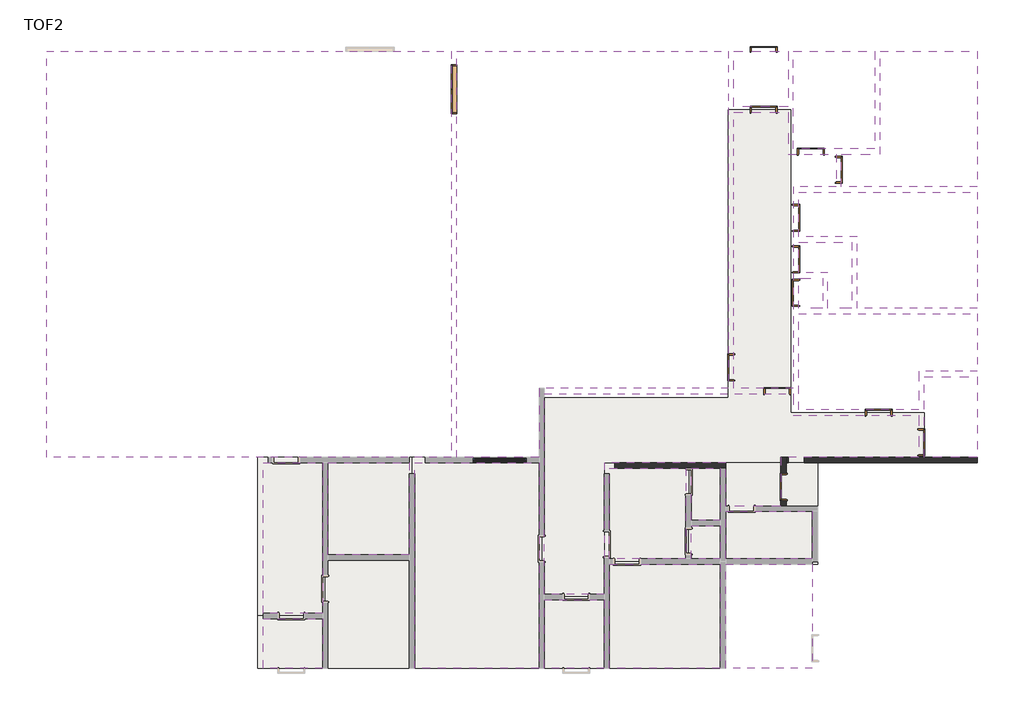
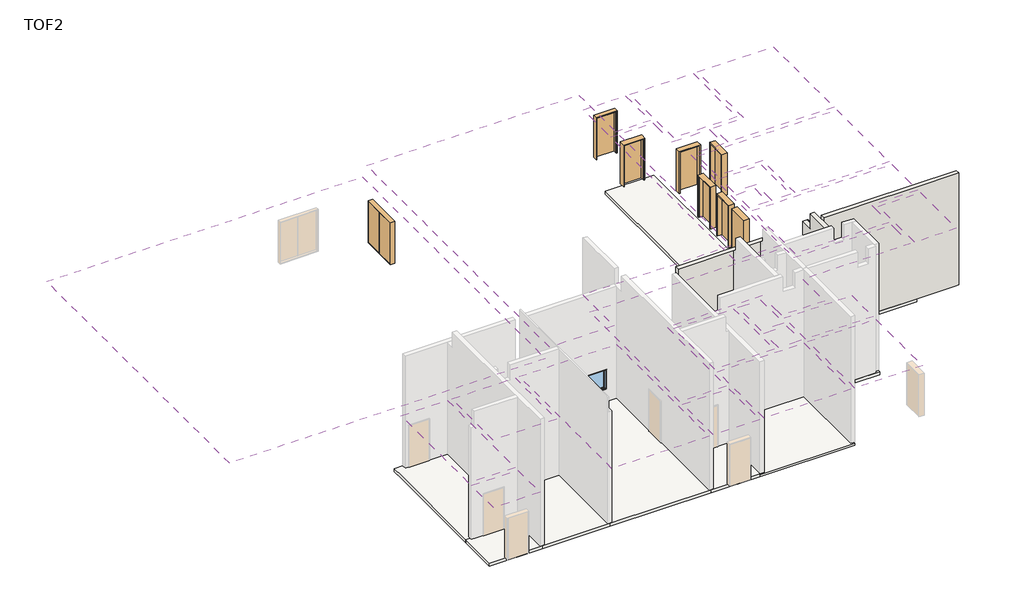
# One storey, part 2 of 2: 23 coverings, 13 doors, 12 slabs, 3 walls, 1 window.
"""IFC4 building model written with IfcOpenShell, lengths in millimetres."""

import ifcopenshell
import ifcopenshell.guid

model = None  # the IFC model being written
_history = None  # IfcOwnerHistory: only IFC2X3 demands one
_inside = {}  # id of a spatial element -> (the spatial element, [elements in it])
_under = {}  # id of a project, library or spatial element -> (it, [spatial elements below it])
_declared = {}  # id of a project -> (the project, [libraries it declares])
_typed = {}  # id of a type object -> (the type object, [elements of that type])
_made_of = {}  # id of a material, layer set ... -> (it, [elements and type objects made of it])


def new_model(schema):
    """Start an empty IFC model of exactly this schema.

    Asked for "IFC4X3", IfcOpenShell would pick the latest addendum, in which some entities
    have other attributes; the version numbers below select the first issue.
    IFC2X3 requires an IfcOwnerHistory on every rooted entity: one is made here for all.
    """
    global model, _history
    if schema == "IFC4X3":
        model = ifcopenshell.file(schema_version=(4, 3, 0, 0))
    else:
        model = ifcopenshell.file(schema=schema)
    _inside.clear()
    _under.clear()
    _declared.clear()
    _typed.clear()
    _made_of.clear()
    _history = None
    if model.schema == "IFC2X3":
        org = make("IfcOrganization", Name="unknown")
        user = make(
            "IfcPersonAndOrganization",
            ThePerson=make("IfcPerson", FamilyName="unknown"),
            TheOrganization=org,
        )
        app = make(
            "IfcApplication",
            ApplicationDeveloper=org,
            Version="unknown",
            ApplicationFullName="unknown",
            ApplicationIdentifier="unknown",
        )
        _history = make(
            "IfcOwnerHistory",
            OwningUser=user,
            OwningApplication=app,
            ChangeAction="ADDED",
            CreationDate=0,
        )
    return model


def make(cls, **values):
    """One entity of the class cls with the attributes given. An attribute that is None is left unset."""
    return model.create_entity(
        cls, **{name: value for name, value in values.items() if value is not None}
    )


def rooted(cls, **values):
    """An entity with a GlobalId (a new one), such as an element, a storey or a relation."""
    return make(cls, GlobalId=ifcopenshell.guid.new(), OwnerHistory=_history, **values)


def si_unit(unit_type, name, prefix=None):
    """IfcSIUnit, for example si_unit("LENGTHUNIT", "METRE", prefix="MILLI")."""
    return make("IfcSIUnit", UnitType=unit_type, Prefix=prefix, Name=name)


def assignment(units):
    """IfcUnitAssignment: the units of a project."""
    return None if units is None else make("IfcUnitAssignment", Units=units)


def point(xyz):
    """IfcCartesianPoint."""
    return None if xyz is None else make("IfcCartesianPoint", Coordinates=xyz)


def direction(xyz):
    """IfcDirection."""
    return None if xyz is None else make("IfcDirection", DirectionRatios=xyz)


def frame(location, z_axis=None, x_axis=None):
    """IfcAxis2Placement3D, a coordinate frame: its origin and axes. An axis left out is left unset."""
    return make(
        "IfcAxis2Placement3D",
        Location=point(location),
        Axis=direction(z_axis),
        RefDirection=direction(x_axis),
    )


def origin():
    """The frame at (0, 0, 0) with its axes left unset."""
    return frame((0.0, 0.0, 0.0))


def origin_with_axes():
    """The frame at (0, 0, 0) with the z axis (0, 0, 1) and the x axis (1, 0, 0) written out."""
    return frame((0.0, 0.0, 0.0), z_axis=(0.0, 0.0, 1.0), x_axis=(1.0, 0.0, 0.0))


def place(relative_to, where):
    """IfcLocalPlacement: puts the frame where relative to a parent placement (None: the world)."""
    return make(
        "IfcLocalPlacement", PlacementRelTo=relative_to, RelativePlacement=where
    )


def context(
    kind, dimensions, precision=None, world=None, true_north=None, identifier=None
):
    """IfcGeometricRepresentationContext, for example the 3D "Model" context."""
    return make(
        "IfcGeometricRepresentationContext",
        ContextIdentifier=identifier,
        ContextType=kind,
        CoordinateSpaceDimension=dimensions,
        Precision=precision,
        WorldCoordinateSystem=world,
        TrueNorth=true_north,
    )


def project(units=None, contexts=None):
    """IfcProject with its units and contexts."""
    return rooted(
        "IfcProject",
        Name="project",
        RepresentationContexts=contexts,
        UnitsInContext=assignment(units),
    )


def spatial(cls, under=None, at=None, **own):
    """A site, building, storey or space (cls), placed at a placement, below another one or the project."""
    s = rooted(cls, ObjectPlacement=at, **own)
    if under is not None:
        _under.setdefault(under.id(), (under, []))[1].append(s)
    return s


def polyline(points):
    """IfcPolyline through the points."""
    return make("IfcPolyline", Points=[point(p) for p in points])


def outline(outer, holes=None, kind="AREA"):
    """IfcArbitraryClosedProfileDef: a profile drawn as a closed curve; with holes, ...WithVoids."""
    if holes is None:
        return make("IfcArbitraryClosedProfileDef", ProfileType=kind, OuterCurve=outer)
    return make(
        "IfcArbitraryProfileDefWithVoids",
        ProfileType=kind,
        OuterCurve=outer,
        InnerCurves=holes,
    )


def extrude(swept, where, along, depth):
    """IfcExtrudedAreaSolid: the profile swept, set in the frame where, extruded along a direction by depth."""
    return make(
        "IfcExtrudedAreaSolid",
        SweptArea=swept,
        Position=where,
        ExtrudedDirection=direction(along),
        Depth=depth,
    )


def faces_of(points, faces, orient=None, outer=None):
    """IfcFace entities. A face is a list of loops; a loop is a list of indices into points, from 0.

    orient and outer hold one flag for each loop. By default every Orientation is true, the
    first loop of a face is its IfcFaceOuterBound and the others are IfcFaceBound.
    """
    made = []
    for i, loops in enumerate(faces):
        bounds = []
        for j, loop in enumerate(loops):
            is_outer = j == 0 if outer is None else outer[i][j]
            bounds.append(
                make(
                    "IfcFaceOuterBound" if is_outer else "IfcFaceBound",
                    Bound=make("IfcPolyLoop", Polygon=[points[k] for k in loop]),
                    Orientation=True if orient is None else orient[i][j],
                )
            )
        made.append(make("IfcFace", Bounds=bounds))
    return made


def faceted_brep(points, faces, orient=None, outer=None, voids=None):
    """IfcFacetedBrep: a solid bounded by flat faces; with voids (closed shells), ...WithVoids."""
    shared = [point(p) for p in points]
    hull = make("IfcClosedShell", CfsFaces=faces_of(shared, faces, orient, outer))
    if voids is None:
        return make("IfcFacetedBrep", Outer=hull)
    return make(
        "IfcFacetedBrepWithVoids",
        Outer=hull,
        Voids=[
            make(cls, CfsFaces=faces_of(shared, fs, o, b)) for cls, fs, o, b in voids
        ],
    )


def shape(context_of_items, identifier, shape_type, items):
    """IfcShapeRepresentation: the items that make up one representation, for example the "Body"."""
    return make(
        "IfcShapeRepresentation",
        ContextOfItems=context_of_items,
        RepresentationIdentifier=identifier,
        RepresentationType=shape_type,
        Items=items,
    )


def source(mapping_origin, context_of_items, identifier, shape_type, items):
    """IfcRepresentationMap: a shape defined once, which mapped items show again and again."""
    return make(
        "IfcRepresentationMap",
        MappingOrigin=mapping_origin,
        MappedRepresentation=shape(context_of_items, identifier, shape_type, items),
    )


def transform(
    local_origin,
    x_axis=None,
    y_axis=None,
    z_axis=None,
    scale=None,
    scale2=None,
    scale3=None,
    uniform=True,
):
    """IfcCartesianTransformationOperator3D, or its non-uniform kind. x_axis, y_axis, z_axis: its Axis1, 2, 3."""
    if uniform:
        return make(
            "IfcCartesianTransformationOperator3D",
            Axis1=direction(x_axis),
            Axis2=direction(y_axis),
            LocalOrigin=point(local_origin),
            Scale=scale,
            Axis3=direction(z_axis),
        )
    return make(
        "IfcCartesianTransformationOperator3DnonUniform",
        Axis1=direction(x_axis),
        Axis2=direction(y_axis),
        LocalOrigin=point(local_origin),
        Scale=scale,
        Axis3=direction(z_axis),
        Scale2=scale2,
        Scale3=scale3,
    )


def mapped(mapping_source, mapping_target):
    """IfcMappedItem: shows the shape of a source again, moved by a transform."""
    return make(
        "IfcMappedItem", MappingSource=mapping_source, MappingTarget=mapping_target
    )


def made_of(thing, what):
    """Note that an element or type object is made of a material, layer set ...; save() writes the relation."""
    if what is not None:
        _made_of.setdefault(what.id(), (what, []))[1].append(thing)
    return thing


def element(
    cls,
    number,
    at=None,
    inside=None,
    cuts=None,
    type_object=None,
    material=None,
    context=None,
    identifier="Body",
    shape_type=None,
    held_by="IfcProductDefinitionShape",
    body=None,
    shapes=None,
    **own,
):
    """One element of the class cls, such as IfcWall. Its Tag is "e" and its number.

    at: its placement. inside: the storey or other place that contains it. cuts: it is an
    opening in that element (IfcRelVoidsElement). A single representation is given by context,
    identifier, shape_type and body (its items); several are given by shapes. held_by: the class
    of the entity that holds the representations. save() writes the other relations.
    """
    e = rooted(cls, Tag="e%d" % number, ObjectPlacement=at, **own)
    if body is not None:
        shapes = [shape(context, identifier, shape_type, body)]
    if shapes is not None:
        e.Representation = make(held_by, Representations=shapes)
    if inside is not None:
        _inside.setdefault(inside.id(), (inside, []))[1].append(e)
    if cuts is not None:
        rooted(
            "IfcRelVoidsElement", RelatingBuildingElement=cuts, RelatedOpeningElement=e
        )
    if type_object is not None:
        _typed.setdefault(type_object.id(), (type_object, []))[1].append(e)
    return made_of(e, material)


def aggregate(whole, parts):
    """IfcRelAggregates: a whole, such as a stair, and the parts it consists of."""
    return rooted("IfcRelAggregates", RelatingObject=whole, RelatedObjects=parts)


def save(model, path):
    """Write the relations noted so far, then the file.

    IfcRelAggregates (storeys below a building ...), IfcRelContainedInSpatialStructure (elements
    in a storey), IfcRelDefinesByType, IfcRelAssociatesMaterial and IfcRelDeclares: one each for
    every whole, place, type object, material and project.
    """
    for whole, parts in _under.values():
        aggregate(whole, parts)
    for where, things in _inside.values():
        rooted(
            "IfcRelContainedInSpatialStructure",
            RelatedElements=things,
            RelatingStructure=where,
        )
    for kind, things in _typed.values():
        rooted("IfcRelDefinesByType", RelatedObjects=things, RelatingType=kind)
    for what, things in _made_of.values():
        rooted("IfcRelAssociatesMaterial", RelatedObjects=things, RelatingMaterial=what)
    for by, libraries in _declared.values():
        rooted("IfcRelDeclares", RelatingContext=by, RelatedDefinitions=libraries)
    model.write(path)


def double_door_steel_22a565f0(model_context):
    return source(origin(), model_context, "Body", "SolidModel", [
        extrude(outline(polyline([(880.0, 60.0), (0.0, 60.0), (0.0, 100.0), (880.0, 100.0), (880.0, 60.0)])), frame((0.0, 0.0, 20.0), z_axis=(0.0, 0.0, 1.0), x_axis=(1.0, 0.0, 0.0)), (0.0, 0.0, 1.0), 2060.0),
        extrude(outline(polyline([(0.0, 60.0), (-880.0, 60.0), (-880.0, 100.0), (0.0, 100.0), (0.0, 60.0)])), frame((0.0, 0.0, 20.0), z_axis=(0.0, 0.0, 1.0), x_axis=(1.0, 0.0, 0.0)), (0.0, 0.0, 1.0), 2060.0),
        faceted_brep([(900.0, -100.0, 2100.0), (900.0, 100.0, 2100.0), (-900.0, 100.0, 2100.0), (-900.0, -100.0, 2100.0), (865.0, 60.0, 2065.0), (865.0, -100.0, 2065.0), (-865.0, -100.0, 2065.0), (-865.0, 60.0, 2065.0), (880.0, 100.0, 2080.0), (880.0, 60.0, 2080.0), (-880.0, 60.0, 2080.0), (-880.0, 100.0, 2080.0), (-900.0, 100.0, 0.0), (-900.0, -100.0, 0.0), (-865.0, -100.0, 35.0), (-865.0, 60.0, 35.0), (-880.0, 60.0, 20.0), (-880.0, 100.0, 20.0), (900.0, 100.0, 0.0), (880.0, 100.0, 20.0), (900.0, -100.0, 0.0), (865.0, -100.0, 35.0), (865.0, 60.0, 35.0), (880.0, 60.0, 20.0)], [[[0, 1, 2, 3]], [[4, 5, 6, 7]], [[8, 9, 10, 11]], [[3, 2, 12, 13]], [[7, 6, 14, 15]], [[11, 10, 16, 17]], [[18, 12, 2, 1], [8, 11, 17, 19]], [[13, 12, 18, 20]], [[0, 3, 13, 20], [21, 14, 6, 5]], [[15, 14, 21, 22]], [[23, 16, 10, 9], [4, 7, 15, 22]], [[17, 16, 23, 19]], [[20, 18, 1, 0]], [[22, 21, 5, 4]], [[19, 23, 9, 8]]]),
    ])


def single_door_steel_02f153ad(model_context):
    return source(origin(), model_context, "Body", "SolidModel", [
        extrude(outline(polyline([(470.0, -130.0), (-470.0, -130.0), (-470.0, -95.0), (470.0, -95.0), (470.0, -130.0)])), origin_with_axes(), (0.0, 0.0, 1.0), 2070.0),
        faceted_brep([(470.0, -130.0, 0.0), (470.0, -95.0, 0.0), (450.0, -95.0, 0.0), (450.0, 95.0, 0.0), (470.0, 95.0, 0.0), (470.0, 130.0, 0.0), (500.0, 130.0, 0.0), (500.0, -130.0, 0.0), (500.0, -130.0, 2100.0), (-500.0, -130.0, 2100.0), (-500.0, -130.0, 0.0), (-470.0, -130.0, 0.0), (-470.0, -130.0, 2070.0), (470.0, -130.0, 2070.0), (500.0, 130.0, 2100.0), (470.0, 130.0, 2070.0), (-470.0, 130.0, 2070.0), (-470.0, 130.0, 0.0), (-500.0, 130.0, 0.0), (-500.0, 130.0, 2100.0), (470.0, 95.0, 2070.0), (450.0, 95.0, 2050.0), (-450.0, 95.0, 2050.0), (-450.0, 95.0, 0.0), (-470.0, 95.0, 0.0), (-470.0, 95.0, 2070.0), (450.0, -95.0, 2050.0), (470.0, -95.0, 2070.0), (-470.0, -95.0, 2070.0), (-470.0, -95.0, 0.0), (-450.0, -95.0, 0.0), (-450.0, -95.0, 2050.0)], [[[0, 1, 2, 3, 4, 5, 6, 7]], [[7, 8, 9, 10, 11, 12, 13, 0]], [[6, 14, 8, 7]], [[5, 15, 16, 17, 18, 19, 14, 6]], [[4, 20, 15, 5]], [[3, 21, 22, 23, 24, 25, 20, 4]], [[2, 26, 21, 3]], [[1, 27, 28, 29, 30, 31, 26, 2]], [[0, 13, 27, 1]], [[12, 11, 29, 28]], [[11, 10, 18, 17, 24, 23, 30, 29]], [[19, 18, 10, 9]], [[25, 24, 17, 16]], [[31, 30, 23, 22]], [[14, 19, 9, 8]], [[20, 25, 16, 15]], [[26, 31, 22, 21]], [[13, 12, 28, 27]]]),
    ])


def single_door_steel_4a6c7de9(model_context):
    return source(origin(), model_context, "Body", "SolidModel", [
        extrude(outline(polyline([(470.0, 130.0), (470.0, 95.0), (-470.0, 95.0), (-470.0, 130.0), (470.0, 130.0)])), origin_with_axes(), (0.0, 0.0, 1.0), 2070.0),
        faceted_brep([(470.0, 130.0, 0.0), (500.0, 130.0, 0.0), (500.0, -130.0, 0.0), (470.0, -130.0, 0.0), (470.0, -95.0, 0.0), (450.0, -95.0, 0.0), (450.0, 95.0, 0.0), (470.0, 95.0, 0.0), (470.0, 130.0, 2070.0), (-470.0, 130.0, 2070.0), (-470.0, 130.0, 0.0), (-500.0, 130.0, 0.0), (-500.0, 130.0, 2100.0), (500.0, 130.0, 2100.0), (500.0, -130.0, 2100.0), (-500.0, -130.0, 2100.0), (-500.0, -130.0, 0.0), (-470.0, -130.0, 0.0), (-470.0, -130.0, 2070.0), (470.0, -130.0, 2070.0), (470.0, -95.0, 2070.0), (-470.0, -95.0, 2070.0), (-470.0, -95.0, 0.0), (-450.0, -95.0, 0.0), (-450.0, -95.0, 2050.0), (450.0, -95.0, 2050.0), (450.0, 95.0, 2050.0), (-450.0, 95.0, 2050.0), (-450.0, 95.0, 0.0), (-470.0, 95.0, 0.0), (-470.0, 95.0, 2070.0), (470.0, 95.0, 2070.0)], [[[0, 1, 2, 3, 4, 5, 6, 7]], [[1, 0, 8, 9, 10, 11, 12, 13]], [[2, 1, 13, 14]], [[3, 2, 14, 15, 16, 17, 18, 19]], [[4, 3, 19, 20]], [[5, 4, 20, 21, 22, 23, 24, 25]], [[6, 5, 25, 26]], [[7, 6, 26, 27, 28, 29, 30, 31]], [[0, 7, 31, 8]], [[9, 30, 29, 10]], [[10, 29, 28, 23, 22, 17, 16, 11]], [[15, 12, 11, 16]], [[21, 18, 17, 22]], [[27, 24, 23, 28]], [[14, 13, 12, 15]], [[20, 19, 18, 21]], [[26, 25, 24, 27]], [[8, 31, 30, 9]]]),
    ])


def single_door_steel_8d57826b(model_context):
    return source(origin(), model_context, "Body", "SolidModel", [
        extrude(outline(polyline([(470.0, -105.0), (-470.0, -105.0), (-470.0, -70.0), (470.0, -70.0), (470.0, -105.0)])), origin_with_axes(), (0.0, 0.0, 1.0), 2070.0),
        faceted_brep([(470.0, -105.0, 0.0), (470.0, -70.0, 0.0), (450.0, -70.0, 0.0), (450.0, 70.0, 0.0), (470.0, 70.0, 0.0), (470.0, 105.0, 0.0), (500.0, 105.0, 0.0), (500.0, -105.0, 0.0), (500.0, -105.0, 2100.0), (-500.0, -105.0, 2100.0), (-500.0, -105.0, 0.0), (-470.0, -105.0, 0.0), (-470.0, -105.0, 2070.0), (470.0, -105.0, 2070.0), (500.0, 105.0, 2100.0), (470.0, 105.0, 2070.0), (-470.0, 105.0, 2070.0), (-470.0, 105.0, 0.0), (-500.0, 105.0, 0.0), (-500.0, 105.0, 2100.0), (470.0, 70.0, 2070.0), (450.0, 70.0, 2050.0), (-450.0, 70.0, 2050.0), (-450.0, 70.0, 0.0), (-470.0, 70.0, 0.0), (-470.0, 70.0, 2070.0), (450.0, -70.0, 2050.0), (470.0, -70.0, 2070.0), (-470.0, -70.0, 2070.0), (-470.0, -70.0, 0.0), (-450.0, -70.0, 0.0), (-450.0, -70.0, 2050.0)], [[[0, 1, 2, 3, 4, 5, 6, 7]], [[7, 8, 9, 10, 11, 12, 13, 0]], [[6, 14, 8, 7]], [[5, 15, 16, 17, 18, 19, 14, 6]], [[4, 20, 15, 5]], [[3, 21, 22, 23, 24, 25, 20, 4]], [[2, 26, 21, 3]], [[1, 27, 28, 29, 30, 31, 26, 2]], [[0, 13, 27, 1]], [[12, 11, 29, 28]], [[11, 10, 18, 17, 24, 23, 30, 29]], [[19, 18, 10, 9]], [[25, 24, 17, 16]], [[31, 30, 23, 22]], [[14, 19, 9, 8]], [[20, 25, 16, 15]], [[26, 31, 22, 21]], [[13, 12, 28, 27]]]),
    ])


def sliding_window_5e64f0fd(model_context):
    return source(origin(), model_context, "Body", "SolidModel", [
        extrude(outline(polyline([(920.0, 27.5), (25.0, 27.5), (25.0, 32.5), (920.0, 32.5), (920.0, 27.5)])), frame((0.0, 0.0, 680.0), z_axis=(0.0, 0.0, 1.0), x_axis=(1.0, 0.0, 0.0)), (0.0, 0.0, 1.0), 840.0),
        extrude(outline(polyline([(-25.0, -32.5), (-920.0, -32.5), (-920.0, -27.5), (-25.0, -27.5), (-25.0, -32.5)])), frame((0.0, 0.0, 680.0), z_axis=(0.0, 0.0, 1.0), x_axis=(1.0, 0.0, 0.0)), (0.0, 0.0, 1.0), 840.0),
        extrude(outline(polyline([(630.0, -970.0), (630.0, 25.0), (1570.0, 25.0), (1570.0, -970.0), (630.0, -970.0)]), holes=[polyline([(1520.0, -920.0), (1520.0, -25.0), (680.0, -25.0), (680.0, -920.0), (1520.0, -920.0)])]), frame((0.0, -55.0, 0.0), z_axis=(0.0, 1.0, 0.0), x_axis=(0.0, 0.0, 1.0)), (0.0, 0.0, 1.0), 47.5),
        extrude(outline(polyline([(630.0, -25.0), (630.0, 970.0), (1570.0, 970.0), (1570.0, -25.0), (630.0, -25.0)]), holes=[polyline([(1520.0, 25.0), (1520.0, 920.0), (680.0, 920.0), (680.0, 25.0), (1520.0, 25.0)])]), frame((0.0, 7.5, 0.0), z_axis=(0.0, 1.0, 0.0), x_axis=(0.0, 0.0, 1.0)), (0.0, 0.0, 1.0), 45.0),
        faceted_brep([(-1000.0, 75.0, 1600.0), (-1000.0, 75.0, 600.0), (-1000.0, -75.0, 600.0), (-1000.0, -75.0, 1600.0), (1000.0, 75.0, 1600.0), (1000.0, 75.0, 600.0), (950.0, 75.0, 650.0), (950.0, 75.0, 1550.0), (-950.0, 75.0, 1550.0), (-950.0, 75.0, 650.0), (1000.0, -75.0, 600.0), (1000.0, -75.0, 1600.0), (-950.0, -75.0, 1550.0), (950.0, -75.0, 1550.0), (950.0, -75.0, 650.0), (-950.0, -75.0, 650.0), (950.0, 55.0, 650.0), (950.0, 55.0, 1550.0), (-950.0, 55.0, 1550.0), (-950.0, 55.0, 1570.0), (-950.0, 5.0, 1570.0), (-950.0, 5.0, 1550.0), (-950.0, -5.0, 1550.0), (-950.0, -5.0, 650.0), (-950.0, 5.0, 650.0), (-950.0, 5.0, 630.0), (-950.0, 55.0, 630.0), (-950.0, 55.0, 650.0), (950.0, -5.0, 650.0), (950.0, 5.0, 650.0), (950.0, -5.0, 630.0), (950.0, -55.0, 630.0), (950.0, -55.0, 650.0), (950.0, -55.0, 1550.0), (950.0, -55.0, 1570.0), (950.0, -5.0, 1570.0), (950.0, -5.0, 1550.0), (950.0, 5.0, 1550.0), (970.0, 5.0, 1570.0), (970.0, 5.0, 630.0), (-970.0, -5.0, 1570.0), (-970.0, -5.0, 630.0), (970.0, 55.0, 1570.0), (970.0, 55.0, 630.0), (-970.0, -55.0, 630.0), (-950.0, -55.0, 1550.0), (-950.0, -55.0, 650.0), (-970.0, -55.0, 1570.0)], [[[0, 1, 2, 3]], [[4, 5, 1, 0], [6, 7, 8, 9]], [[1, 5, 10, 2]], [[10, 11, 3, 2], [12, 13, 14, 15]], [[7, 6, 16, 17]], [[9, 8, 18, 19, 20, 21, 22, 23, 24, 25, 26, 27]], [[16, 6, 9, 27]], [[5, 4, 11, 10]], [[28, 29, 24, 23]], [[28, 30, 31, 32, 14, 13, 33, 34, 35, 36, 37, 29]], [[29, 37, 21, 20, 38, 39, 25, 24]], [[40, 41, 30, 28, 23, 22, 36, 35]], [[39, 38, 42, 43]], [[39, 43, 26, 25]], [[43, 42, 19, 18, 17, 16, 27, 26]], [[41, 44, 31, 30]], [[45, 46, 32, 31, 44, 47, 34, 33]], [[46, 15, 14, 32]], [[12, 15, 46, 45]], [[47, 44, 41, 40]], [[3, 11, 4, 0]], [[7, 17, 18, 8]], [[37, 36, 22, 21]], [[42, 38, 20, 19]], [[12, 45, 33, 13]], [[47, 40, 35, 34]]]),
    ])


model = new_model("IFC4")

# Units and contexts
model_context = context("Model", 3, world=origin())
ifc_project = project(units=[si_unit("LENGTHUNIT", "METRE", prefix="MILLI")], contexts=[model_context])

# Site, building, storey
site = spatial("IfcSite", under=ifc_project)
building = spatial("IfcBuilding", under=site)
storey = spatial("IfcBuildingStorey", under=building, Name="TOF2", Elevation=1149.9618634)

# Coverings
placement = place(None, origin())
element("IfcCovering", 1, ObjectType="H_CE_AR_B09_Acoustic Ceiling_T Bar_600x600x9T", at=placement, inside=storey, context=model_context, shape_type="SweptSolid", body=[
    extrude(outline(polyline([(18300.0, 8599.5208589), (18300.0, 23599.5208589), (33250.0, 23599.5208589), (33250.0, 8599.5208589), (18300.0, 8599.5208589)])), frame((0.0, 0.0, 4149.9618634), z_axis=(0.0, 0.0, 1.0), x_axis=(1.0, 0.0, 0.0)), (0.0, 0.0, 1.0), 9.0),
])
element("IfcCovering", 2, ObjectType="H_CE_AR_B09_Acoustic Ceiling_T Bar_600x600x9T", at=placement, inside=storey, context=model_context, shape_type="SweptSolid", body=[
    extrude(outline(polyline([(33450.0, 8599.5208589), (33450.0, 23599.5208589), (43500.0, 23599.5208589), (43500.0, 11149.5208589), (36500.0, 11149.5208589), (36500.0, 8599.5208589), (33450.0, 8599.5208589)])), frame((0.0, 0.0, 4649.9618634), z_axis=(0.0, 0.0, 1.0), x_axis=(1.0, 0.0, 0.0)), (0.0, 0.0, 1.0), 9.0),
])
element("IfcCovering", 3, ObjectType="H_CE_AR_B09_Acoustic Ceiling_T Bar_600x600x9T", at=placement, inside=storey, context=model_context, shape_type="SweptSolid", body=[
    extrude(outline(polyline([(43700.0, 23599.5208589), (45700.0, 23599.5208589), (45700.0, 21549.5208589), (43700.0, 21549.5208589), (43700.0, 23599.5208589)])), frame((0.0, 0.0, 3849.9618634), z_axis=(0.0, 0.0, 1.0), x_axis=(1.0, 0.0, 0.0)), (0.0, 0.0, 1.0), 9.0),
])
element("IfcCovering", 4, ObjectType="H_CE_AR_B09_Acoustic Ceiling_T Bar_600x600x9T", at=placement, inside=storey, context=model_context, shape_type="SweptSolid", body=[
    extrude(outline(polyline([(45900.0, 23599.5208589), (48900.0, 23599.5208589), (48900.0, 19999.5208589), (45900.0, 19999.5208589), (45900.0, 23599.5208589)])), frame((0.0, 0.0, 3849.9618634), z_axis=(0.0, 0.0, 1.0), x_axis=(1.0, 0.0, 0.0)), (0.0, 0.0, 1.0), 9.0),
])
element("IfcCovering", 5, ObjectType="H_CE_AR_B09_Acoustic Ceiling_T Bar_600x600x9T", at=placement, inside=storey, context=model_context, shape_type="SweptSolid", body=[
    extrude(outline(polyline([(49100.0, 23599.5208589), (52700.0, 23599.5208589), (52700.0, 18599.5208589), (47675.0, 18599.5208589), (47675.0, 19799.5208589), (49100.0, 19799.5208589), (49100.0, 23599.5208589)])), frame((0.0, 0.0, 3849.9618634), z_axis=(0.0, 0.0, 1.0), x_axis=(1.0, 0.0, 0.0)), (0.0, 0.0, 1.0), 9.0),
])
element("IfcCovering", 6, ObjectType="H_CE_AR_B09_Acoustic Ceiling_T Bar_600x600x9T", at=placement, inside=storey, context=model_context, shape_type="SweptSolid", body=[
    extrude(outline(polyline([(45895.0, 18599.5208589), (45895.0, 11149.5208589), (43700.0, 11149.5208589), (43700.0, 21349.5208589), (45700.0, 21349.5208589), (45700.0, 19799.5208589), (47475.0, 19799.5208589), (47475.0, 18599.5208589), (45895.0, 18599.5208589)])), frame((0.0, 0.0, 3849.9618634), z_axis=(0.0, 0.0, 1.0), x_axis=(1.0, 0.0, 0.0)), (0.0, 0.0, 1.0), 9.0),
])
element("IfcCovering", 7, ObjectType="H_CE_AR_B09_Acoustic Ceiling_T Bar_600x600x9T", at=placement, inside=storey, context=model_context, shape_type="SweptSolid", body=[
    extrude(outline(polyline([(52700.0, 18399.5208589), (52700.0, 14099.5208589), (48250.0, 14099.5208589), (48250.0, 16749.5208589), (46095.0, 16749.5208589), (46095.0, 18399.5208589), (52700.0, 18399.5208589)])), frame((0.0, 0.0, 3849.9618634), z_axis=(0.0, 0.0, 1.0), x_axis=(1.0, 0.0, 0.0)), (0.0, 0.0, 1.0), 9.0),
])
element("IfcCovering", 8, ObjectType="H_CE_AR_B09_Acoustic Ceiling_T Bar_600x600x9T", at=placement, inside=storey, context=model_context, shape_type="SweptSolid", body=[
    extrude(outline(polyline([(47175.0, 15414.5208589), (46095.0, 15414.5208589), (46095.0, 16549.5208589), (48050.0, 16549.5208589), (48050.0, 14099.5208589), (47175.0, 14099.5208589), (47175.0, 15414.5208589)])), frame((0.0, 0.0, 3849.9618634), z_axis=(0.0, 0.0, 1.0), x_axis=(1.0, 0.0, 0.0)), (0.0, 0.0, 1.0), 9.0),
])
element("IfcCovering", 9, ObjectType="H_CE_AR_B09_Acoustic Ceiling_T Bar_600x600x9T", at=placement, inside=storey, context=model_context, shape_type="SweptSolid", body=[
    extrude(outline(polyline([(46975.0, 14099.5208589), (46095.0, 14099.5208589), (46095.0, 15214.5208589), (46975.0, 15214.5208589), (46975.0, 14099.5208589)])), frame((0.0, 0.0, 3849.9618634), z_axis=(0.0, 0.0, 1.0), x_axis=(1.0, 0.0, 0.0)), (0.0, 0.0, 1.0), 9.0),
])
element("IfcCovering", 10, ObjectType="H_CE_AR_B09_Acoustic Ceiling_T Bar_600x600x9T", at=placement, inside=storey, context=model_context, shape_type="SweptSolid", body=[
    extrude(outline(polyline([(52700.0, 13899.5208589), (52700.0, 11774.5208589), (50525.0, 11774.5208589), (50525.0, 10349.5208589), (46095.0, 10349.5208589), (46095.0, 13899.5208589), (52700.0, 13899.5208589)])), frame((0.0, 0.0, 3849.9618634), z_axis=(0.0, 0.0, 1.0), x_axis=(1.0, 0.0, 0.0)), (0.0, 0.0, 1.0), 9.0),
])
element("IfcCovering", 11, ObjectType="H_CE_AR_B09_Acoustic Ceiling_T Bar_600x600x9T", at=placement, inside=storey, context=model_context, shape_type="SweptSolid", body=[
    extrude(outline(polyline([(52700.0, 11574.5208589), (52700.0, 8599.5208589), (50725.0, 8599.5208589), (50725.0, 11574.5208589), (52700.0, 11574.5208589)])), frame((0.0, 0.0, 3849.9618634), z_axis=(0.0, 0.0, 1.0), x_axis=(1.0, 0.0, 0.0)), (0.0, 0.0, 1.0), 9.0),
])
element("IfcCovering", 12, ObjectType="H_CE_AR_B09_Acoustic Ceiling_T Bar_600x600x9T", at=placement, inside=storey, context=model_context, shape_type="SweptSolid", body=[
    extrude(outline(polyline([(38900.0, 3543.8249516), (36700.0, 3543.8249516), (36700.0, 10949.5208589), (45895.0, 10949.5208589), (45895.0, 10149.5208589), (50525.0, 10149.5208589), (50525.0, 8599.5208589), (45440.0, 8599.5208589), (45440.0, 6799.5208589), (43400.0, 6799.5208589), (43400.0, 8404.5208589), (38900.0, 8404.5208589), (38900.0, 3543.8249516)])), frame((0.0, 0.0, 3849.9618634), z_axis=(0.0, 0.0, 1.0), x_axis=(1.0, 0.0, 0.0)), (0.0, 0.0, 1.0), 9.0),
])
element("IfcCovering", 13, ObjectType="H_CE_AR_B09_Acoustic Ceiling_T Bar_600x600x9T", at=placement, inside=storey, context=model_context, shape_type="SweptSolid", body=[
    extrude(outline(polyline([(46600.0, 4649.5208589), (46600.0, 799.5208589), (43400.0, 799.5208589), (43400.0, 4649.5208589), (46600.0, 4649.5208589)])), frame((0.0, 0.0, 3849.9618634), z_axis=(0.0, 0.0, 1.0), x_axis=(1.0, 0.0, 0.0)), (0.0, 0.0, 1.0), 9.0),
])
element("IfcCovering", 14, ObjectType="H_CE_AR_B09_Acoustic Ceiling_T Bar_600x600x9T", at=placement, inside=storey, context=model_context, shape_type="SweptSolid", body=[
    extrude(outline(polyline([(46600.0, 4849.5208589), (43400.0, 4849.5208589), (43400.0, 6599.5208589), (46600.0, 6599.5208589), (46600.0, 4849.5208589)])), frame((0.0, 0.0, 3849.9618634), z_axis=(0.0, 0.0, 1.0), x_axis=(1.0, 0.0, 0.0)), (0.0, 0.0, 1.0), 9.0),
])
element("IfcCovering", 15, ObjectType="H_CE_AR_B09_Acoustic Ceiling_T Bar_600x600x9T", at=placement, inside=storey, context=model_context, shape_type="SweptSolid", body=[
    extrude(outline(polyline([(43200.0, 6074.5208589), (43200.0, 4849.5208589), (42125.0, 4849.5208589), (42125.0, 6074.5208589), (43200.0, 6074.5208589)])), frame((0.0, 0.0, 3849.9618634), z_axis=(0.0, 0.0, 1.0), x_axis=(1.0, 0.0, 0.0)), (0.0, 0.0, 1.0), 9.0),
])
element("IfcCovering", 16, ObjectType="H_CE_AR_B09_Acoustic Ceiling_T Bar_600x600x9T", at=placement, inside=storey, context=model_context, shape_type="SweptSolid", body=[
    extrude(outline(polyline([(42125.0, 6274.5208589), (42125.0, 8204.5208589), (43200.0, 8204.5208589), (43200.0, 6274.5208589), (42125.0, 6274.5208589)])), frame((0.0, 0.0, 3849.9618634), z_axis=(0.0, 0.0, 1.0), x_axis=(1.0, 0.0, 0.0)), (0.0, 0.0, 1.0), 9.0),
])
element("IfcCovering", 17, ObjectType="H_CE_AR_B09_Acoustic Ceiling_T Bar_600x600x9T", at=placement, inside=storey, context=model_context, shape_type="SweptSolid", body=[
    extrude(outline(polyline([(39100.0, 4849.5208589), (39100.0, 8204.5208589), (41925.0, 8204.5208589), (41925.0, 4849.5208589), (39100.0, 4849.5208589)])), frame((0.0, 0.0, 3849.9618634), z_axis=(0.0, 0.0, 1.0), x_axis=(1.0, 0.0, 0.0)), (0.0, 0.0, 1.0), 9.0),
])
element("IfcCovering", 18, ObjectType="H_CE_AR_B09_Acoustic Ceiling_T Bar_600x600x9T", at=placement, inside=storey, context=model_context, shape_type="SweptSolid", body=[
    extrude(outline(polyline([(43200.0, 4649.5208589), (43200.0, 799.5208589), (39100.0, 799.5208589), (39100.0, 4649.5208589), (43200.0, 4649.5208589)])), frame((0.0, 0.0, 3849.9618634), z_axis=(0.0, 0.0, 1.0), x_axis=(1.0, 0.0, 0.0)), (0.0, 0.0, 1.0), 9.0),
])
element("IfcCovering", 19, ObjectType="H_CE_AR_B09_Acoustic Ceiling_T Bar_600x600x9T", at=placement, inside=storey, context=model_context, shape_type="SweptSolid", body=[
    extrude(outline(polyline([(38900.0, 3343.8249516), (38900.0, 799.5208589), (36700.0, 799.5208589), (36700.0, 3343.8249516), (38900.0, 3343.8249516)])), frame((0.0, 0.0, 3849.9618634), z_axis=(0.0, 0.0, 1.0), x_axis=(1.0, 0.0, 0.0)), (0.0, 0.0, 1.0), 9.0),
])
element("IfcCovering", 20, ObjectType="H_CE_AR_B09_Acoustic Ceiling_T Bar_600x600x9T", at=placement, inside=storey, context=model_context, shape_type="SweptSolid", body=[
    extrude(outline(polyline([(36500.0, 799.5208589), (31900.0, 799.5208589), (31900.0, 8399.5208589), (36500.0, 8399.5208589), (36500.0, 799.5208589)])), frame((0.0, 0.0, 3849.9618634), z_axis=(0.0, 0.0, 1.0), x_axis=(1.0, 0.0, 0.0)), (0.0, 0.0, 1.0), 9.0),
])
element("IfcCovering", 21, ObjectType="H_CE_AR_B09_Acoustic Ceiling_T Bar_600x600x9T", at=placement, inside=storey, context=model_context, shape_type="SweptSolid", body=[
    extrude(outline(polyline([(28700.0, 4999.0208589), (28700.0, 8399.5208589), (31700.0, 8399.5208589), (31700.0, 4999.0208589), (28700.0, 4999.0208589)])), frame((0.0, 0.0, 3849.9618634), z_axis=(0.0, 0.0, 1.0), x_axis=(1.0, 0.0, 0.0)), (0.0, 0.0, 1.0), 9.0),
])
element("IfcCovering", 22, ObjectType="H_CE_AR_B09_Acoustic Ceiling_T Bar_600x600x9T", at=placement, inside=storey, context=model_context, shape_type="SweptSolid", body=[
    extrude(outline(polyline([(26300.0, 2837.0208589), (26300.0, 8399.5208589), (28500.0, 8399.5208589), (28500.0, 2837.0208589), (26300.0, 2837.0208589)])), frame((0.0, 0.0, 3849.9618634), z_axis=(0.0, 0.0, 1.0), x_axis=(1.0, 0.0, 0.0)), (0.0, 0.0, 1.0), 9.0),
])
element("IfcCovering", 23, ObjectType="H_CE_AR_B09_Acoustic Ceiling_T Bar_600x600x9T", at=placement, inside=storey, context=model_context, shape_type="SweptSolid", body=[
    extrude(outline(polyline([(28500.0, 799.5208589), (26300.0, 799.5208589), (26300.0, 2637.0208589), (28500.0, 2637.0208589), (28500.0, 799.5208589)])), frame((0.0, 0.0, 3849.9618634), z_axis=(0.0, 0.0, 1.0), x_axis=(1.0, 0.0, 0.0)), (0.0, 0.0, 1.0), 9.0),
])

# Doors
double_door_steel_shape = double_door_steel_22a565f0(model_context)
element("IfcDoor", 24, ObjectType="Double Door_Steel : H_DR_AR_B12_Double Door_Steel_W2000xH2100", at=placement, inside=storey, context=model_context, shape_type="MappedRepresentation", body=[
    mapped(double_door_steel_shape, transform((33350.0, 22199.5208589, 1149.9618634), x_axis=(0.0, 1.0, 0.0), y_axis=(-1.0, 0.0, 0.0), z_axis=(0.0, 0.0, 1.0))),
])
single_door_steel_shape = single_door_steel_02f153ad(model_context)
element("IfcDoor", 25, ObjectType="Single Door_Steel : H_DR_AR_B12_Single Door_Steel_W1000xH2100", at=placement, inside=storey, context=model_context, shape_type="MappedRepresentation", body=[
    mapped(single_door_steel_shape, transform((44800.0, 21449.5208589, 1149.9618634), x_axis=(-1.0, 0.0, 0.0), y_axis=(0.0, -1.0, 0.0), z_axis=(0.0, 0.0, 1.0))),
])
element("IfcDoor", 26, ObjectType="Single Door_Steel : H_DR_AR_B12_Single Door_Steel_W1000xH2100", at=placement, inside=storey, context=model_context, shape_type="MappedRepresentation", body=[
    mapped(single_door_steel_shape, transform((47575.0, 19224.5208589, 1149.9618634), x_axis=(0.0, 1.0, 0.0), y_axis=(-1.0, 0.0, 0.0), z_axis=(0.0, 0.0, 1.0))),
])
element("IfcDoor", 27, ObjectType="Single Door_Steel : H_DR_AR_B12_Single Door_Steel_W1000xH2100", at=placement, inside=storey, context=model_context, shape_type="MappedRepresentation", body=[
    mapped(single_door_steel_shape, transform((45300.0, 11049.5208589, 1149.9618634), x_axis=(-1.0, 0.0, 0.0), y_axis=(0.0, -1.0, 0.0), z_axis=(0.0, 0.0, 1.0))),
])
element("IfcDoor", 28, ObjectType="Single Door_Steel : H_DR_AR_B12_Single Door_Steel_W1000xH2100", at=placement, inside=storey, context=model_context, shape_type="MappedRepresentation", body=[
    mapped(single_door_steel_shape, transform((50625.0, 9149.5208589, 1149.9618634), x_axis=(0.0, 1.0, 0.0), y_axis=(-1.0, 0.0, 0.0), z_axis=(0.0, 0.0, 1.0))),
])
single_door_steel_2_shape = single_door_steel_4a6c7de9(model_context)
element("IfcDoor", 29, ObjectType="Single Door_Steel : H_DR_AR_B12_Single Door_Steel_W1000xH2100", at=placement, inside=storey, context=model_context, shape_type="MappedRepresentation", body=[
    mapped(single_door_steel_2_shape, transform((43600.0, 11924.5208589, 1149.9618634), x_axis=(0.0, 1.0, 0.0), y_axis=(-1.0, 0.0, 0.0), z_axis=(0.0, 0.0, 1.0))),
])
element("IfcDoor", 30, ObjectType="Single Door_Steel : H_DR_AR_B12_Single Door_Steel_W1000xH2100", at=placement, inside=storey, context=model_context, shape_type="MappedRepresentation", body=[
    mapped(single_door_steel_2_shape, transform((46545.0, 19899.5208589, 1149.9618634), x_axis=(1.0, 0.0, 0.0), y_axis=(0.0, 1.0, 0.0), z_axis=(0.0, 0.0, 1.0))),
])
element("IfcDoor", 31, ObjectType="Single Door_Steel : H_DR_AR_B12_Single Door_Steel_W1000xH2100", at=placement, inside=storey, context=model_context, shape_type="MappedRepresentation", body=[
    mapped(single_door_steel_2_shape, transform((45995.0, 17449.5208589, 1149.9618634), x_axis=(0.0, -1.0, 0.0), y_axis=(1.0, 0.0, 0.0), z_axis=(0.0, 0.0, 1.0))),
])
element("IfcDoor", 32, ObjectType="Single Door_Steel : H_DR_AR_B12_Single Door_Steel_W1000xH2100", at=placement, inside=storey, context=model_context, shape_type="MappedRepresentation", body=[
    mapped(single_door_steel_2_shape, transform((45995.0, 15912.0208589, 1149.9618634), x_axis=(0.0, -1.0, 0.0), y_axis=(1.0, 0.0, 0.0), z_axis=(0.0, 0.0, 1.0))),
])
element("IfcDoor", 33, ObjectType="Single Door_Steel : H_DR_AR_B12_Single Door_Steel_W1000xH2100", at=placement, inside=storey, context=model_context, shape_type="MappedRepresentation", body=[
    mapped(single_door_steel_2_shape, transform((49050.0, 10249.5208589, 1149.9618634), x_axis=(1.0, 0.0, 0.0), y_axis=(0.0, 1.0, 0.0), z_axis=(0.0, 0.0, 1.0))),
])
element("IfcDoor", 34, ObjectType="Single Door_Steel : H_DR_AR_B12_Single Door_Steel_W1000xH2100", at=placement, inside=storey, context=model_context, shape_type="MappedRepresentation", body=[
    mapped(single_door_steel_2_shape, transform((45540.0, 7503.8249516, 1149.9618634), x_axis=(0.0, 1.0, 0.0), y_axis=(-1.0, 0.0, 0.0), z_axis=(0.0, 0.0, 1.0))),
])
element("IfcDoor", 35, ObjectType="Single Door_Steel : H_DR_AR_B12_Single Door_Steel_W1000xH2100", at=placement, inside=storey, context=model_context, shape_type="MappedRepresentation", body=[
    mapped(single_door_steel_2_shape, transform((45995.0, 14674.5208589, 1149.9618634), x_axis=(0.0, 1.0, 0.0), y_axis=(-1.0, 0.0, 0.0), z_axis=(0.0, 0.0, 1.0))),
])
single_door_steel_3_shape = single_door_steel_8d57826b(model_context)
element("IfcDoor", 36, ObjectType="Single Door_Steel : H_DR_AR_B12_Single Door_Steel_W1000xH2100", at=placement, inside=storey, context=model_context, shape_type="MappedRepresentation", body=[
    mapped(single_door_steel_3_shape, transform((44800.0, 23674.5208589, 1149.9618634), x_axis=(-1.0, 0.0, 0.0), y_axis=(0.0, -1.0, 0.0), z_axis=(0.0, 0.0, 1.0))),
])

# Slabs
element("IfcSlab", 37, ObjectType="H_SF_AR_S17_SOG T150_GS1", at=placement, inside=storey, context=model_context, shape_type="Brep", body=[
    faceted_brep([(26100.0, 2737.0208589, 999.9618634), (26100.0, 7999.5208589, 999.9618634), (26100.0, 8599.5208589, 999.9618634), (26500.0, 8599.5208589, 999.9618634), (28600.0, 8599.5208589, 999.9618634), (28600.0, 8399.5208589, 999.9618634), (28600.0, 4899.0208589, 999.9618634), (28600.0, 2737.0208589, 999.9618634), (26300.0, 2737.0208589, 999.9618634), (26100.0, 2737.0208589, 1149.9618634), (26300.0, 2737.0208589, 1149.9618634), (28600.0, 2737.0208589, 1149.9618634), (28600.0, 4899.0208589, 1149.9618634), (28600.0, 8399.5208589, 1149.9618634), (28600.0, 8599.5208589, 1149.9618634), (27650.0, 8599.5208589, 1149.9618634), (26650.0, 8599.5208589, 1149.9618634), (26500.0, 8599.5208589, 1149.9618634), (26100.0, 8599.5208589, 1149.9618634), (26100.0, 7999.5208589, 1149.9618634)], [[[0, 1, 2, 3, 4, 5, 6, 7, 8]], [[9, 10, 11, 12, 13, 14, 15, 16, 17, 18, 19]], [[2, 1, 0, 9, 19, 18]], [[4, 3, 2, 18, 17, 16, 15, 14]], [[7, 6, 5, 4, 14, 13, 12, 11]], [[0, 8, 7, 11, 10, 9]]]),
])
element("IfcSlab", 38, ObjectType="H_SF_AR_S17_SOG T150_GS1", at=placement, inside=storey, context=model_context, shape_type="SweptSolid", body=[
    extrude(outline(polyline([(26100.0, 2737.0208589), (28600.0, 2737.0208589), (28600.0, 799.5208589), (26100.0, 799.5208589), (26100.0, 2737.0208589)])), frame((0.0, 0.0, 999.9618634), z_axis=(0.0, 0.0, 1.0), x_axis=(1.0, 0.0, 0.0)), (0.0, 0.0, 1.0), 150.0),
])
element("IfcSlab", 39, ObjectType="H_SF_AR_S17_SOG T150_GS1", at=placement, inside=storey, context=model_context, shape_type="SweptSolid", body=[
    extrude(outline(polyline([(28600.0, 8599.5208589), (31800.0, 8599.5208589), (31800.0, 4899.0208589), (28600.0, 4899.0208589), (28600.0, 8599.5208589)])), frame((0.0, 0.0, 999.9618634), z_axis=(0.0, 0.0, 1.0), x_axis=(1.0, 0.0, 0.0)), (0.0, 0.0, 1.0), 150.0),
])
element("IfcSlab", 40, ObjectType="H_SF_AR_S17_SOG T150_GS1", at=placement, inside=storey, context=model_context, shape_type="Brep", body=[
    faceted_brep([(28600.0, 4899.0208589, 999.9618634), (31800.0, 4899.0208589, 999.9618634), (31800.0, 799.5208589, 999.9618634), (28600.0, 799.5208589, 999.9618634), (28600.0, 2737.0208589, 999.9618634), (28600.0, 4899.0208589, 1149.9618634), (28600.0, 2737.0208589, 1149.9618634), (28600.0, 799.5208589, 1149.9618634), (31800.0, 799.5208589, 1149.9618634), (31800.0, 4899.0208589, 1149.9618634)], [[[0, 1, 2, 3, 4]], [[5, 6, 7, 8, 9]], [[1, 0, 5, 9]], [[2, 1, 9, 8]], [[3, 2, 8, 7]], [[0, 4, 3, 7, 6, 5]]]),
])
element("IfcSlab", 41, ObjectType="H_SF_AR_S17_SOG T150_GS1", at=placement, inside=storey, context=model_context, shape_type="Brep", body=[
    faceted_brep([(31800.0, 8599.5208589, 999.9618634), (36600.0, 8599.5208589, 999.9618634), (36600.0, 3443.8249516, 999.9618634), (36600.0, 799.5208589, 999.9618634), (31800.0, 799.5208589, 999.9618634), (31800.0, 4899.0208589, 999.9618634), (31800.0, 8599.5208589, 1149.9618634), (31800.0, 4899.0208589, 1149.9618634), (31800.0, 799.5208589, 1149.9618634), (36600.0, 799.5208589, 1149.9618634), (36600.0, 3443.8249516, 1149.9618634), (36600.0, 8599.5208589, 1149.9618634)], [[[0, 1, 2, 3, 4, 5]], [[6, 7, 8, 9, 10, 11]], [[1, 0, 6, 11]], [[3, 2, 1, 11, 10, 9]], [[4, 3, 9, 8]], [[0, 5, 4, 8, 7, 6]]]),
])
element("IfcSlab", 42, ObjectType="H_SF_AR_S17_SOG T150_GS1", at=placement, inside=storey, context=model_context, shape_type="Brep", body=[
    faceted_brep([(38900.0, 3443.8249516, 999.9618634), (38900.0, 799.5208589, 999.9618634), (36600.0, 799.5208589, 999.9618634), (36600.0, 3443.8249516, 999.9618634), (38900.0, 3443.8249516, 1149.9618634), (36600.0, 3443.8249516, 1149.9618634), (36600.0, 799.5208589, 1149.9618634), (38900.0, 799.5208589, 1149.9618634), (38900.0, 799.5208589, 1099.9618634)], [[[0, 1, 2, 3]], [[4, 5, 6, 7]], [[1, 0, 4, 7, 8]], [[2, 1, 8, 7, 6]], [[3, 2, 6, 5]], [[0, 3, 5, 4]]]),
])
element("IfcSlab", 43, ObjectType="H_SF_AR_S17_SOG T150_GS1", at=placement, inside=storey, context=model_context, shape_type="Brep", body=[
    faceted_brep([(36600.0, 3443.8249516, 999.9618634), (36600.0, 8599.5208589, 999.9618634), (36600.0, 10799.5208589, 999.9618634), (36700.0, 10799.5208589, 999.9618634), (43500.0, 10799.5208589, 999.9618634), (43500.0, 21449.5208589, 999.9618634), (45800.0, 21449.5208589, 999.9618634), (45800.0, 10249.5208589, 999.9618634), (50725.0, 10249.5208589, 999.9618634), (50725.0, 8404.5208589, 999.9618634), (46800.0, 8404.5208589, 999.9618634), (43400.0, 8404.5208589, 999.9618634), (42025.0, 8404.5208589, 999.9618634), (38900.0, 8404.5208589, 999.9618634), (38900.0, 4749.5208589, 999.9618634), (38900.0, 3443.8249516, 999.9618634), (36600.0, 3443.8249516, 1149.9618634), (38900.0, 3443.8249516, 1149.9618634), (38900.0, 8404.5208589, 1149.9618634), (43400.0, 8404.5208589, 1149.9618634), (46800.0, 8404.5208589, 1149.9618634), (50725.0, 8404.5208589, 1149.9618634), (50725.0, 10249.5208589, 1149.9618634), (45800.0, 10249.5208589, 1149.9618634), (45800.0, 21449.5208589, 1149.9618634), (43500.0, 21449.5208589, 1149.9618634), (43500.0, 10799.5208589, 1149.9618634), (36600.0, 10799.5208589, 1149.9618634), (36600.0, 8599.5208589, 1149.9618634), (38900.0, 8404.5208589, 1099.9618634)], [[[0, 1, 2, 3, 4, 5, 6, 7, 8, 9, 10, 11, 12, 13, 14, 15]], [[16, 17, 18, 19, 20, 21, 22, 23, 24, 25, 26, 27, 28]], [[15, 14, 13, 29, 18, 17]], [[0, 15, 17, 16]], [[2, 1, 0, 16, 28, 27]], [[4, 3, 2, 27, 26]], [[5, 4, 26, 25]], [[6, 5, 25, 24]], [[7, 6, 24, 23]], [[8, 7, 23, 22]], [[9, 8, 22, 21]], [[13, 12, 11, 10, 9, 21, 20, 19, 18, 29]]]),
])
element("IfcSlab", 44, ObjectType="H_SF_AR_S17_SOG T100_GS1", at=placement, inside=storey, context=model_context, shape_type="Brep", body=[
    faceted_brep([(38900.0, 4749.5208589, 999.9618634), (38900.0, 8404.5208589, 999.9618634), (42025.0, 8404.5208589, 999.9618634), (42025.0, 6174.5208589, 999.9618634), (42025.0, 4749.5208589, 999.9618634), (38900.0, 8404.5208589, 1099.9618634), (38900.0, 4749.5208589, 1099.9618634), (42025.0, 4749.5208589, 1099.9618634), (42025.0, 6174.5208589, 1099.9618634), (42025.0, 8404.5208589, 1099.9618634)], [[[0, 1, 2, 3, 4]], [[5, 6, 7, 8, 9]], [[1, 0, 6, 5]], [[2, 1, 5, 9]], [[4, 3, 2, 9, 8, 7]], [[0, 4, 7, 6]]]),
])
element("IfcSlab", 45, ObjectType="H_SF_AR_S17_SOG T100_GS1", at=placement, inside=storey, context=model_context, shape_type="SweptSolid", body=[
    extrude(outline(polyline([(42025.0, 8404.5208589), (43400.0, 8404.5208589), (43400.0, 6174.5208589), (42025.0, 6174.5208589), (42025.0, 8404.5208589)])), frame((0.0, 0.0, 999.9618634), z_axis=(0.0, 0.0, 1.0), x_axis=(1.0, 0.0, 0.0)), (0.0, 0.0, 1.0), 100.0),
])
element("IfcSlab", 46, ObjectType="H_SF_AR_S17_SOG T100_GS1", at=placement, inside=storey, context=model_context, shape_type="SweptSolid", body=[
    extrude(outline(polyline([(43400.0, 6174.5208589), (43400.0, 4749.5208589), (42025.0, 4749.5208589), (42025.0, 6174.5208589), (43400.0, 6174.5208589)])), frame((0.0, 0.0, 999.9618634), z_axis=(0.0, 0.0, 1.0), x_axis=(1.0, 0.0, 0.0)), (0.0, 0.0, 1.0), 100.0),
])
element("IfcSlab", 47, ObjectType="H_SF_AR_S17_SOG T100_GS1", at=placement, inside=storey, context=model_context, shape_type="Brep", body=[
    faceted_brep([(38900.0, 4749.5208589, 999.9618634), (42025.0, 4749.5208589, 999.9618634), (43400.0, 4749.5208589, 999.9618634), (43400.0, 4649.5208589, 999.9618634), (43400.0, 799.5208589, 999.9618634), (38900.0, 799.5208589, 999.9618634), (38900.0, 3443.8249516, 999.9618634), (43400.0, 4749.5208589, 1099.9618634), (42025.0, 4749.5208589, 1099.9618634), (38900.0, 4749.5208589, 1099.9618634), (38900.0, 3443.8249516, 1099.9618634), (38900.0, 799.5208589, 1099.9618634), (43400.0, 799.5208589, 1099.9618634)], [[[0, 1, 2, 3, 4, 5, 6]], [[7, 8, 9, 10, 11, 12]], [[9, 0, 6, 5, 11, 10]], [[2, 1, 0, 9, 8, 7]], [[4, 3, 2, 7, 12]], [[5, 4, 12, 11]]]),
])
element("IfcSlab", 48, ObjectType="H_SF_AR_S17_SOG T150_GS1", at=placement, inside=storey, context=model_context, shape_type="Brep", body=[
    faceted_brep([(46800.0, 8404.5208589, 999.9618634), (46800.0, 4649.5208589, 999.9618634), (43400.0, 4649.5208589, 999.9618634), (43400.0, 4749.5208589, 999.9618634), (43400.0, 6174.5208589, 999.9618634), (43400.0, 8404.5208589, 999.9618634), (46800.0, 4649.5208589, 1149.9618634), (46800.0, 8404.5208589, 1149.9618634), (43400.0, 8404.5208589, 1149.9618634), (43400.0, 4649.5208589, 1149.9618634), (43400.0, 8404.5208589, 1099.9618634)], [[[0, 1, 2, 3, 4, 5]], [[6, 7, 8, 9]], [[1, 0, 7, 6]], [[2, 1, 6, 9]], [[5, 4, 3, 2, 9, 8, 10]], [[0, 5, 10, 8, 7]]]),
])

# Walls
element("IfcWall", 49, ObjectType="H_WA_AR_B02_Int Wall_Block T200", at=placement, inside=storey, context=model_context, shape_type="Brep", body=[
    faceted_brep([(39300.0, 8204.5208589, 1149.9618634), (41925.0, 8204.5208589, 1149.9618634), (42125.0, 8204.5208589, 1149.9618634), (43200.0, 8204.5208589, 1149.9618634), (43400.0, 8204.5208589, 1149.9618634), (43400.0, 8204.5208589, 6749.9618634), (42125.0, 8204.5208589, 6749.9618634), (41925.0, 8204.5208589, 6749.9618634), (39300.0, 8204.5208589, 6749.9618634), (43400.0, 8404.5208589, 1149.9618634), (39300.0, 8404.5208589, 1149.9618634), (39300.0, 8404.5208589, 6749.9618634), (43400.0, 8404.5208589, 6749.9618634)], [[[0, 1, 2, 3, 4, 5, 6, 7, 8]], [[9, 10, 11, 12]], [[9, 4, 3, 2, 1, 0, 10]], [[4, 9, 12, 5]], [[10, 0, 8, 11]], [[8, 7, 6, 5, 12, 11]]]),
])
element("IfcWall", 50, ObjectType="H_WA_AR_B02_Int Wall_Block T200", at=placement, inside=storey, context=model_context, shape_type="Brep", body=[
    faceted_brep([(45440.0, 8003.8249516, 1149.9618634), (45440.0, 8003.8249516, 3249.9618634), (45440.0, 7003.8249516, 3249.9618634), (45440.0, 7003.8249516, 1149.9618634), (45440.0, 6799.5208589, 1149.9618634), (45440.0, 6799.5208589, 7499.9618634), (45440.0, 7999.5208589, 7499.9618634), (45440.0, 7999.5208589, 6749.9618634), (45440.0, 8599.5208589, 6749.9618634), (45440.0, 8599.5208589, 1149.9618634), (45640.0, 8003.8249516, 3249.9618634), (45640.0, 8003.8249516, 1149.9618634), (45640.0, 8399.5208589, 1149.9618634), (45640.0, 8599.5208589, 1149.9618634), (45640.0, 8599.5208589, 6749.9618634), (45640.0, 8399.5208589, 6749.9618634), (45640.0, 7999.5208589, 6749.9618634), (45640.0, 7999.5208589, 7499.9618634), (45640.0, 6799.5208589, 7499.9618634), (45640.0, 6799.5208589, 1149.9618634), (45640.0, 7003.8249516, 1149.9618634), (45640.0, 7003.8249516, 3249.9618634)], [[[0, 1, 2, 3, 4, 5, 6, 7, 8, 9]], [[10, 11, 12, 13, 14, 15, 16, 17, 18, 19, 20, 21]], [[19, 4, 3, 20]], [[9, 13, 12, 11, 0]], [[4, 19, 18, 5]], [[13, 9, 8, 14]], [[10, 1, 0, 11]], [[1, 10, 21, 2]], [[2, 21, 20, 3]], [[16, 7, 6, 17]], [[7, 16, 15, 14, 8]], [[6, 5, 18, 17]]]),
])
element("IfcWall", 51, ObjectType="H_WA_AR_B02_Int Wall_Block T200", at=placement, inside=storey, context=model_context, shape_type="Brep", body=[
    faceted_brep([(45640.0, 8399.5208589, 1149.9618634), (45700.0, 8399.5208589, 1149.9618634), (45700.0, 8399.5208589, 6749.9618634), (45640.0, 8399.5208589, 6749.9618634), (45700.0, 8599.5208589, 1149.9618634), (45640.0, 8599.5208589, 1149.9618634), (45640.0, 8599.5208589, 6749.9618634), (45700.0, 8599.5208589, 6749.9618634)], [[[0, 1, 2, 3]], [[4, 5, 6, 7]], [[0, 5, 4, 1]], [[5, 0, 3, 6]], [[1, 4, 7, 2]], [[3, 2, 7, 6]]]),
    faceted_brep([(46300.0, 8399.5208589, 1149.9618634), (52574.0, 8399.5208589, 1149.9618634), (52700.0, 8399.5208589, 1149.9618634), (52700.0, 8399.5208589, 6749.9618634), (52574.0, 8399.5208589, 6749.9618634), (46300.0, 8399.5208589, 6749.9618634), (52700.0, 8599.5208589, 1149.9618634), (52574.0, 8599.5208589, 1149.9618634), (46300.0, 8599.5208589, 1149.9618634), (46300.0, 8599.5208589, 6749.9618634), (52700.0, 8599.5208589, 6749.9618634)], [[[0, 1, 2, 3, 4, 5]], [[6, 7, 8, 9, 10]], [[6, 2, 1, 0, 8, 7]], [[2, 6, 10, 3]], [[8, 0, 5, 9]], [[5, 4, 3, 10, 9]]]),
])

# Window
sliding_window_shape = sliding_window_5e64f0fd(model_context)
element("IfcWindow", 52, ObjectType="Sliding Window : H_WD_AR_B11_Sliding_Steel Window_DG_W2000xH1000", at=placement, inside=storey, context=model_context, shape_type="MappedRepresentation", body=[
    mapped(sliding_window_shape, transform((35050.0, 8499.5208589, 1149.9618634), x_axis=(-1.0, 0.0, 0.0), y_axis=(0.0, -1.0, 0.0), z_axis=(0.0, 0.0, 1.0))),
])

save(model, "model.ifc")

# Revit data of these elements
# Type "H_CE_AR_B09_Acoustic Ceiling_T Bar_600x600x9T"
#   built-in parameter 1002203 = 1 (stored number, unit not read)
#   built-in parameter 1002202 = 1 (stored number, unit not read)
#   Layers, outside or top first: 9 mm no material (function 4)
# Type "Double Door_Steel : H_DR_AR_B12_Double Door_Steel_W2000xH2100"
#   Type Mark = ""
#   프레임 = ""
#   철물 = ""
#   유리/마감 = ""
#   위치/개소 = ""
#   부호 = "1/SD"
#   문번호 = ""
#   문기호 = "SD"
#   Analytic Construction = "<None>"
#   Height = 2100 mm
#   Width = 1800 mm
#   Define Thermal Properties by = 1
#   문 틀 = none
#   문 = none
#   Function = (empty or 0)
#   Assembly Code = ""
#   Wall Closure = (empty or 0)
# Type "Single Door_Steel : H_DR_AR_B12_Single Door_Steel_W1000xH2100"
#   Type Mark = "SD"
#   Analytic Construction = "<None>"
#   프레임 투영 외부. = 25 mm
#   프레임 투영 내부. = 25 mm
#   프레임 폭 = 75 mm
#   Height = 2100 mm
#   Width = 1000 mm
#   Define Thermal Properties by = 1
#   문 패널 = none
#   문 프레임 = none
#   Function = (empty or 0)
#   Wall Closure = (empty or 0)
# Type "H_SF_AR_S17_SOG T150_GS1"
#   Type Comments = "구조_콘크리트"
#   Layers, outside or top first: 150 mm "Concrete - Cast-in-Place Concrete - 35 MPa" (function 1)
# Type "H_SF_AR_S17_SOG T100_GS1"
#   Type Comments = "구조_콘크리트"
#   Layers, outside or top first: 100 mm "Concrete - Cast-in-Place Concrete - 35 MPa" (function 1)
# Type "H_WA_AR_B02_Int Wall_Block T200"
#   Type Comments = ""
#   Layers, outside or top first: 200 mm "00_Masonry_Conc. Block" (function 1)
# Type "Sliding Window : H_WD_AR_B11_Sliding_Steel Window_DG_W2000xH1000"
#   Description = "Steel Frame + 2 x T=6mm + T12mm Air Space"
#   Type Mark = ""
#   Analytic Construction = "<None>"
#   창 두께 = 150 mm
#   Visual Light Transmittance = 0.88
#   Thermal Resistance (R) = 0.271106 (m²·K)/W
#   Solar Heat Gain Coefficient = 0.81
#   Height = 1000 mm
#   Heat Transfer Coefficient (U) = 6.2426 W/(m²·K)
#   기본 씰 높이 = 600 mm
#   Width = 2000 mm
#   Define Thermal Properties by = 1
#   창 패널 = none
#   창 프레임 = none
#   Construction Type Id = ""
#   Wall Closure = (empty or 0)
# Element 1 (IfcCovering, "H_CE_AR_B09_Acoustic Ceiling_T Bar_600x600x9T")
#   Height Offset From Level = 3000 mm
#   Phase Created = New Construction
# Element 2 (IfcCovering, "H_CE_AR_B09_Acoustic Ceiling_T Bar_600x600x9T")
#   Height Offset From Level = 3500 mm
#   Phase Created = New Construction
# Elements 3, 4, 5, 6, 7, 8, 9, 10, 11, 12, 13, 14, 15, 16, 17, 18, 19, 20, 21, 22, 23 (IfcCovering, "H_CE_AR_B09_Acoustic Ceiling_T Bar_600x600x9T")
#   Height Offset From Level = 2700 mm
#   Phase Created = New Construction
# Element 24 (IfcDoor, "Double Door_Steel : H_DR_AR_B12_Double Door_Steel_W2000xH2100")
#   H_Door Style Name = "Steel Door_Double_Transsom"
#   H_Door_Frame = "Steel"
#   H_Door_Leaf = "Steel"
#   H_Door_Vision = "N.A"
#   H_Door_Panic = "N.A"
#   H_Door_Style Remark = ""
#   H_Door_Fire Rating = "NA/0.5/1.0\n/1.5/2.0"
#   H_Door Style No = DDT11
#   Phase Created = New Construction
# Elements 25, 26, 27, 28, 29, 30, 31, 32, 33, 34, 35, 36 (IfcDoor, "Single Door_Steel : H_DR_AR_B12_Single Door_Steel_W1000xH2100")
#   H_Door Style Name = "Steel Door_Single"
#   H_Door_Frame = "Steel"
#   H_Door_Leaf = "Steel"
#   H_Door_Vision = "N.A"
#   H_Door_Panic = "N.A"
#   H_Door_Style Remark = "Steel Door w/ Steel Frame"
#   H_Door_Fire Rating = "NA/0.5/1.0\n/1.5/2.0"
#   H_Door Style No = SD11
#   Phase Created = New Construction
# Element 37 (IfcSlab, "H_SF_AR_S17_SOG T150_GS1")
#   Comments = ""
#   built-in parameter 1001955 = -1.5708 (stored number, unit not read)
#   Height Offset From Level = 0 mm
#   built-in parameter 1001954 = 1
#   Phase Created = New Construction
#   Materials on its faces: "Concrete - Cast-in-Place Concrete - 35 MPa"
# Elements 38, 39, 40, 41, 43 (IfcSlab, "H_SF_AR_S17_SOG T150_GS1")
#   Comments = ""
#   built-in parameter 1001955 = 3.14159 (stored number, unit not read)
#   Height Offset From Level = 0 mm
#   built-in parameter 1001954 = 1
#   Phase Created = New Construction
#   Materials on its faces: "Concrete - Cast-in-Place Concrete - 35 MPa"
# Elements 42, 48 (IfcSlab, "H_SF_AR_S17_SOG T150_GS1")
#   Comments = ""
#   Height Offset From Level = 0 mm
#   built-in parameter 1001954 = 1
#   Phase Created = New Construction
#   Materials on its faces: "Concrete - Cast-in-Place Concrete - 35 MPa"
# Elements 44, 47 (IfcSlab, "H_SF_AR_S17_SOG T100_GS1")
#   Comments = ""
#   built-in parameter 1001955 = -1.5708 (stored number, unit not read)
#   Height Offset From Level = -50 mm
#   built-in parameter 1001954 = 1
#   Phase Created = New Construction
#   Materials on its faces: "Concrete - Cast-in-Place Concrete - 35 MPa"
# Element 45 (IfcSlab, "H_SF_AR_S17_SOG T100_GS1")
#   Comments = ""
#   built-in parameter 1001955 = 3.14159 (stored number, unit not read)
#   Height Offset From Level = -50 mm
#   built-in parameter 1001954 = 1
#   Phase Created = New Construction
#   Materials on its faces: "Concrete - Cast-in-Place Concrete - 35 MPa"
# Element 46 (IfcSlab, "H_SF_AR_S17_SOG T100_GS1")
#   Comments = ""
#   built-in parameter 1001955 = 1.5708 (stored number, unit not read)
#   Height Offset From Level = -50 mm
#   built-in parameter 1001954 = 1
#   Phase Created = New Construction
#   Materials on its faces: "Concrete - Cast-in-Place Concrete - 35 MPa"
# Elements 49, 50, 51 (IfcWall, "H_WA_AR_B02_Int Wall_Block T200")
#   H_Wall Style Name = "Block Wall"
#   H_Wall-Base Material-1 = "Concrete Block"
#   H_Wall-Base Material-2 = ""
